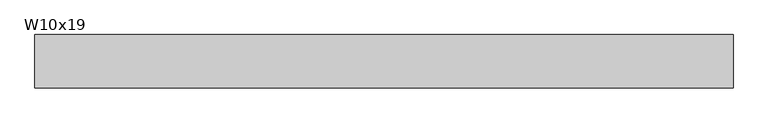
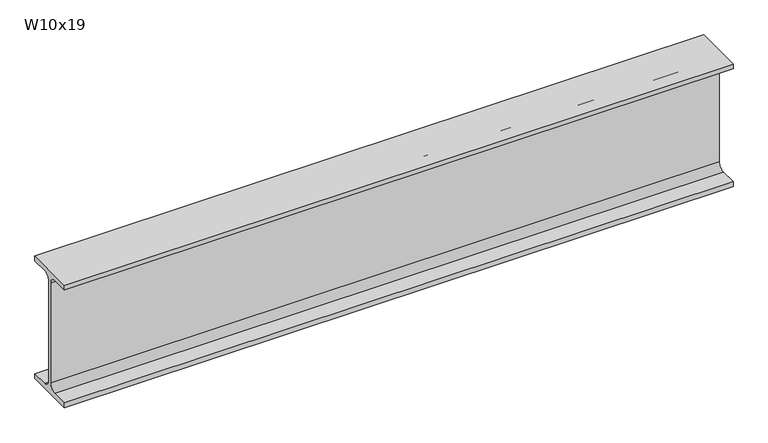
"""IFC4 building model written with IfcOpenShell, lengths in millimetres: beam geometry, RME W-Wide Flange : W10x19."""

from ifc_helpers import new_model, si_unit, point, frame, frame_2d, origin, place, context, project, spatial, polyline, circle_curve, trimmed, segment, composite_curve, outline, extrude, source, transform, mapped, element, save


def w10x19_8393e01b(model_context):
    return source(origin(), model_context, "Body", "SweptSolid", [
        extrude(outline(composite_curve([segment(polyline([(51.054, -119.507), (51.054, -129.54), (-51.054, -129.54), (-51.054, -119.507), (-16.9545, -119.507)]), True, "CONTINUOUS"), segment(trimmed(circle_curve(frame_2d((-16.9545, -105.7275)), 13.7795), [point((-16.9545, -119.507))], [point((-3.175, -105.7275))], True, "CARTESIAN"), True, "CONTINUOUS"), segment(polyline([(-3.175, -105.7275), (-3.175, 105.7275)]), True, "CONTINUOUS"), segment(trimmed(circle_curve(frame_2d((-16.9545, 105.7275)), 13.7795), [point((-3.175, 105.7275))], [point((-16.9545, 119.507))], True, "CARTESIAN"), True, "CONTINUOUS"), segment(polyline([(-16.9545, 119.507), (-51.054, 119.507), (-51.054, 129.54), (51.054, 129.54), (51.054, 119.507), (16.9545, 119.507)]), True, "CONTINUOUS"), segment(trimmed(circle_curve(frame_2d((16.9545, 105.7275)), 13.7795), [point((16.9545, 119.507))], [point((3.175, 105.7275))], True, "CARTESIAN"), True, "CONTINUOUS"), segment(polyline([(3.175, 105.7275), (3.175, -105.7275)]), True, "CONTINUOUS"), segment(trimmed(circle_curve(frame_2d((16.9545, -105.7275)), 13.7795), [point((3.175, -105.7275))], [point((16.9545, -119.507))], True, "CARTESIAN"), True, "CONTINUOUS"), segment(polyline([(16.9545, -119.507), (51.054, -119.507)]), True, "CONTINUOUS")], self_intersect=False)), frame((-624.400409, 0.0, 0.0), z_axis=(1.0, 0.0, 0.0), x_axis=(0.0, 1.0, 0.0)), (0.0, 0.0, 1.0), 1337.700818),
    ])


if __name__ == "__main__":
    model = new_model("IFC4")
    model_context = context("Model", 3, world=origin())
    ifc_project = project(units=[si_unit("LENGTHUNIT", "METRE", prefix="MILLI")], contexts=[model_context])
    site = spatial("IfcSite", under=ifc_project)
    building = spatial("IfcBuilding", under=site)
    placement = place(None, origin())
    w10x19_shape = w10x19_8393e01b(model_context)
    element("IfcBeam", 1, ObjectType="RME W-Wide Flange : W10x19", at=placement, inside=building, context=model_context, shape_type="MappedRepresentation", body=[
        mapped(w10x19_shape, transform((0.0, 0.0, 0.0), x_axis=(1.0, 0.0, 0.0), y_axis=(0.0, 1.0, 0.0), z_axis=(0.0, 0.0, 1.0))),
    ])
    save(model, "model.ifc")

# Revit data of these elements
# Type "RME W-Wide Flange : W10x19"
#   WELD P [instance default] = ""
#   WELD LE [instance default] = ""
#   WELD D [instance default] = ""
#   TOP SECTION SIZE [instance default] = ""
#   TOP SECTION LENGTH [instance default] = ""
#   REMARKS [instance default] = ""
#   REINF TYPE [instance default] = ""
#   Nominal Size = "W24"
#   End Bearing Capacity [instance default] = ""
#   BOT SECTION SIZE [instance default] = ""
#   BOT SECTION LENGTH [instance default] = ""
#   Assembly Code = "B10"
#   W = 19
#   Start Extension Calculation [instance default] = 10' - 0"
#   Start Extension [instance default] = -0' - 0 1/2"
#   End Extension Calculation [instance default] = 10' - 0"
#   End Extension [instance default] = -0' - 0 1/2"
#   Length [instance default] = 5' - 0"
#   bf = 0' - 4.02"
#   d = 0' - 10.2"
#   k = 0' - 0 15/16"
#   k2 = 0' - 0.5425"
#   tf = 0' - 0.395"
#   tw = 0' - 0 1/4"
#   A = 0.0390278 SF
#   Structural Material [instance default] = Metal - Steel - ASTM A992
# Element 1 (IfcBeam, "RME W-Wide Flange : W10x19")
#   Length = 4' - 8.16539"
#   Materials on its faces: "Metal - Steel - ASTM A992"
# Materials
#   "Metal - Steel - ASTM A992": class "Metal", colour RGB 255 128 0, transparency 0
